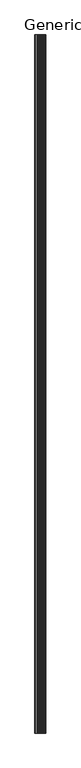
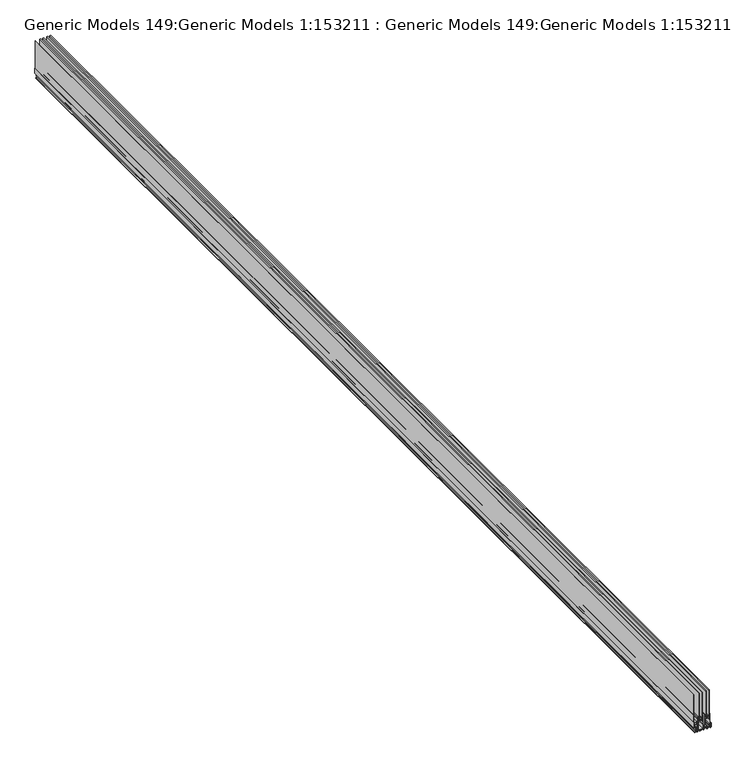
"""IFC4 building model written with IfcOpenShell, lengths in millimetres: proxy geometry, Generic Models 149:Generic Models 1:153211 : Generic Models 149:Generic Models 1:153211."""

from ifc_helpers import new_model, si_unit, frame, origin, place, context, project, spatial, polyline, outline, extrude, source, transform, mapped, element, save


def generic_models_149_generic_models_1_153211_generic_models_8e53df71(model_context):
    return source(origin(), model_context, "Body", "SweptSolid", [
        extrude(outline(polyline([(-6626.7463019, -5303.1974793), (-6626.7463019, 2583.5025207), (-6612.4164704, 2583.5025207), (-6612.4164704, -5303.1974793), (-6626.7463019, -5303.1974793)])), frame((0.0, 0.0, 55.1497405), z_axis=(0.0, 0.0, 1.0), x_axis=(1.0, 0.0, 0.0)), (0.0, 0.0, 1.0), 7.9798298),
        extrude(outline(polyline([(-6611.6227204, -5303.1974793), (-6611.6227204, 2583.5025207), (-6606.8813862, 2583.5025207), (-6606.8813862, -5303.1974793), (-6611.6227204, -5303.1974793)])), frame((0.0, 0.0, 54.3559905), z_axis=(0.0, 0.0, 1.0), x_axis=(1.0, 0.0, 0.0)), (0.0, 0.0, 1.0), 191.9290887),
        extrude(outline(polyline([(-6632.2813862, -5303.1974793), (-6632.2813862, 2583.5025207), (-6627.5400519, 2583.5025207), (-6627.5400519, -5303.1974793), (-6632.2813862, -5303.1974793)])), frame((0.0, 0.0, 54.3559905), z_axis=(0.0, 0.0, 1.0), x_axis=(1.0, 0.0, 0.0)), (0.0, 0.0, 1.0), 191.9290887),
        extrude(outline(polyline([(-6578.4016395, -5303.1974793), (-6578.4016395, 2583.5025207), (-6564.071808, 2583.5025207), (-6564.071808, -5303.1974793), (-6578.4016395, -5303.1974793)])), frame((0.0, 0.0, 55.1497405), z_axis=(0.0, 0.0, 1.0), x_axis=(1.0, 0.0, 0.0)), (0.0, 0.0, 1.0), 7.9798298),
        extrude(outline(polyline([(-15.24, -6644.7273792), (-15.24, -6643.4573766), (37.5919931, -6643.4573766), (37.5919931, -6646.5053852), (43.7726598, -6646.5053852), (43.7726598, -6664.8674677), (246.2850793, -6664.8674677), (246.2850793, -6665.6612177), (43.7726598, -6665.6612177), (43.7726598, -6667.2487177), (7.4338791, -6667.2487177), (4.8675216, -6657.1733817), (-15.2400103, -6657.1733817), (-15.2400103, -6655.9033792), (-2.2860103, -6655.9033792), (-2.2860103, -6644.7273792), (-15.24, -6644.7273792)]), holes=[polyline([(28.2786614, -6654.9720561), (26.5853256, -6654.9720561), (26.5853256, -6644.8120561), (-1.0160111, -6644.8120561), (-1.0160111, -6655.9033905), (5.8846955, -6655.9033905), (8.3602567, -6665.8940484), (12.1073187, -6665.8940484), (12.1073187, -6663.5233922), (13.3773204, -6663.5233922), (13.3773204, -6665.8940622), (36.3219905, -6665.8940622), (36.3219905, -6658.6973955), (42.5026598, -6658.6973955), (42.5026598, -6647.7753766), (36.3219931, -6647.7753766), (36.3219931, -6644.7273955), (28.2786614, -6644.7273955), (28.2786614, -6654.9720561)])]), frame((0.0, -5303.1974793, 0.0), z_axis=(0.0, 1.0, 0.0), x_axis=(0.0, 0.0, 1.0)), (0.0, 0.0, 1.0), 7886.7),
        extrude(outline(polyline([(-6563.278058, -5303.1974793), (-6563.278058, 2583.5025207), (-6558.5367238, 2583.5025207), (-6558.5367238, -5303.1974793), (-6563.278058, -5303.1974793)])), frame((0.0, 0.0, 54.3559905), z_axis=(0.0, 0.0, 1.0), x_axis=(1.0, 0.0, 0.0)), (0.0, 0.0, 1.0), 191.9290887),
        extrude(outline(polyline([(-6583.9367238, -5303.1974793), (-6583.9367238, 2583.5025207), (-6579.1953895, 2583.5025207), (-6579.1953895, -5303.1974793), (-6583.9367238, -5303.1974793)])), frame((0.0, 0.0, 54.3559905), z_axis=(0.0, 0.0, 1.0), x_axis=(1.0, 0.0, 0.0)), (0.0, 0.0, 1.0), 191.9290887),
        extrude(outline(polyline([(0.0, -6550.5780441), (-8.6360103, -6550.5780441), (-8.6360103, -6548.8000502), (-15.3674764, -6548.8000502), (-16.8486778, -6565.6487169), (-20.3200111, -6565.6487169), (-20.3200111, -6564.6327246), (-23.6220034, -6564.6327246), (-23.6220034, -6567.342058), (-22.6906701, -6568.1887246), (-22.0663514, -6569.1788543), (-21.6787466, -6570.1699246), (-21.5376159, -6571.1605246), (-21.6527194, -6572.1492432), (-22.0338174, -6573.1346691), (-22.6906701, -6574.1153913), (-23.6220034, -6575.0467246), (-23.6220034, -6577.7560502), (-20.320013, -6577.7560502), (-20.320013, -6576.7400502), (-17.8646796, -6576.7400502), (-17.8646796, -6580.1267169), (-20.320013, -6580.1267169), (-20.320013, -6602.1400502), (-22.860013, -6602.1400502), (-22.860013, -6605.0187169), (-20.4046796, -6605.0187169), (-20.4046796, -6634.1440502), (-22.860013, -6634.1440502), (-22.860013, -6637.0227169), (-20.4046796, -6637.0227169), (-20.4046796, -6639.4780502), (-27.7706796, -6639.4780502), (-27.7706796, -6649.2147169), (-23.7913463, -6649.2147169), (-23.7913463, -6651.1620502), (-27.7706796, -6651.1620502), (-27.7706796, -6660.6447169), (-31.750013, -6660.6447169), (-31.750013, -6654.2947169), (-30.1413463, -6654.2947169), (-30.1413463, -6641.5100502), (-31.750013, -6641.5100502), (-31.750013, -6637.0227169), (-25.2306796, -6637.0227169), (-25.2306796, -6633.2973835), (-22.860013, -6631.6810199), (-22.860013, -6624.1533905), (-31.7500155, -6624.1533905), (-31.7500155, -6621.6980571), (-29.8026822, -6621.6980571), (-28.0246822, -6620.6820571), (-27.4320198, -6621.2747195), (-26.3664552, -6621.6128724), (-25.1616557, -6621.5016454), (-24.4138082, -6620.853893), (-24.1056981, -6619.9009438), (-24.2201111, -6618.8741262), (-24.7398327, -6618.0047688), (-25.6476485, -6617.5242), (-26.4599658, -6617.5340508), (-27.4320181, -6617.8880511), (-28.0246847, -6618.4807177), (-30.1413514, -6617.2953844), (-29.3793514, -6616.2793844), (-28.528177, -6615.6312532), (-27.6236156, -6615.205372), (-26.6816597, -6614.9998594), (-25.718302, -6615.0128338), (-24.749535, -6615.2424137), (-23.7913514, -6615.6867177), (-22.8600181, -6616.4487177), (-22.8600181, -6607.4740511), (-25.2306847, -6605.7916425), (-25.2306847, -6598.9227177), (-31.7500181, -6598.9227177), (-31.7500181, -6596.5520511), (-23.6220181, -6596.5520511), (-23.6220181, -6580.1267177), (-25.9926847, -6578.4443091), (-25.9926847, -6575.8087177), (-31.7500181, -6575.8087177), (-31.7500181, -6573.4380511), (-30.0566847, -6573.4380511), (-28.0246847, -6572.2527177), (-27.4320181, -6572.9300588), (-26.4101923, -6573.2529926), (-25.2207414, -6573.1319292), (-24.4457934, -6572.4847749), (-24.0882255, -6571.5370539), (-24.1509152, -6570.5142905), (-24.6367399, -6569.6420089), (-25.5485767, -6569.1457332), (-26.3945623, -6569.135145), (-27.4320181, -6569.4587255), (-28.0246847, -6570.1360588), (-30.1413514, -6568.8660588), (-29.3793514, -6567.9347255), (-28.3633514, -6567.1727255), (-27.2626847, -6566.7493922), (-25.9926847, -6566.5800588), (-25.9926847, -6562.2620502), (-18.913985, -6562.2620502), (-17.8105346, -6548.8000441), (-26.924, -6548.8000441), (-26.924, -6551.1707108), (-29.3793333, -6551.1707108), (-29.3793333, -6552.7793775), (-31.75, -6552.7793775), (-31.75, -6548.8000441), (-29.3793333, -6548.8000441), (-29.3793333, -6546.3447108), (0.0, -6546.3447108), (0.0, -6550.5780441)])), frame((0.0, -5303.1974793, 0.0), z_axis=(0.0, 1.0, 0.0), x_axis=(0.0, 0.0, 1.0)), (0.0, 0.0, 1.0), 7886.7),
        extrude(outline(polyline([(-13.8853402, -6587.2387142), (-11.5146736, -6585.0373809), (-11.5146736, -6581.1427117), (-4.5720042, -6581.1427117), (-4.5720042, -6586.0533905), (32.3426624, -6586.0533905), (32.3426624, -6582.8360571), (33.9513291, -6582.8360571), (33.9513291, -6586.0533792), (48.8526537, -6586.0533792), (49.6993204, -6585.8840458), (50.545987, -6585.3760458), (51.053987, -6584.5293792), (51.2233204, -6583.6827125), (51.2233204, -6577.3327125), (51.0539905, -6576.5707125), (49.7937115, -6575.3596656), (48.8208346, -6575.2246403), (47.8761103, -6575.6274864), (47.0746572, -6576.5707125), (46.9053239, -6577.3327125), (46.9053239, -6579.9573792), (45.0426572, -6579.9573792), (45.0426572, -6573.5227125), (47.1593239, -6572.3373792), (47.6673239, -6572.9300571), (48.9341881, -6573.370951), (49.7440381, -6573.2555999), (50.445459, -6572.8014428), (50.9693239, -6571.9987238), (51.1386572, -6571.2367238), (50.969335, -6570.4747255), (50.1126338, -6569.4019675), (49.3483574, -6569.1184329), (48.5102155, -6569.1688264), (47.667335, -6569.5433922), (47.159335, -6570.1360588), (45.0426684, -6568.9507091), (45.0426684, -6562.5160425), (46.905335, -6562.5160425), (46.905335, -6565.1407091), (47.0746537, -6565.9027134), (48.3377549, -6567.1150146), (49.3109454, -6567.2487856), (50.254729, -6566.8443135), (51.053987, -6565.9027134), (51.2233308, -6565.1407134), (51.2233308, -6558.7907238), (51.0539975, -6557.8593905), (50.5459975, -6557.0973905), (49.6993308, -6556.5893905), (48.8526641, -6556.4200571), (33.9513308, -6556.4200571), (33.9513308, -6559.6373905), (32.3426641, -6559.6373905), (32.3426641, -6556.4200571), (-4.5720034, -6556.4200571), (-4.5720034, -6561.3307228), (-10.1600034, -6561.3307228), (-10.1600034, -6554.0493878), (75.0146624, -6554.0493878), (75.0146624, -6556.4200467), (55.964665, -6556.4200467), (55.0333316, -6556.58938), (54.2713316, -6557.09738), (53.7633316, -6557.85938), (53.593988, -6558.7907134), (53.593988, -6583.6827238), (53.7633213, -6584.5293905), (54.2713213, -6585.3760571), (55.0333213, -6585.8840571), (55.9646547, -6586.0533905), (75.0146547, -6586.0533905), (75.0146547, -6588.4240571), (-12.7483988, -6588.4240571), (-15.7480069, -6591.0487142), (-17.6953402, -6593.0807142), (-19.3040069, -6595.2820475), (-17.8646736, -6592.3187142), (-16.0020069, -6589.6940475), (-13.8853402, -6587.2387142)])), frame((0.0, -5303.1974793, 0.0), z_axis=(0.0, 1.0, 0.0), x_axis=(0.0, 0.0, 1.0)), (0.0, 0.0, 1.0), 7886.7),
        extrude(outline(polyline([(32.3426641, -6604.764716), (-22.0133376, -6604.764716), (-22.0133376, -6602.3940502), (75.0146624, -6602.3940502), (75.0146624, -6604.7647091), (55.964665, -6604.7647091), (55.0333316, -6604.9340425), (54.2713316, -6605.4420425), (53.7633316, -6606.2040425), (53.593988, -6607.1353758), (53.593988, -6632.0273862), (53.7633213, -6632.8740529), (54.2713213, -6633.7207196), (55.0333213, -6634.2287196), (55.9646547, -6634.3980529), (75.0146624, -6634.3980529), (75.0146624, -6636.768715), (-22.0133376, -6636.768715), (-22.0133376, -6634.3980614), (32.3426624, -6634.3980614), (32.3426624, -6631.1807196), (33.9513291, -6631.1807196), (33.9513291, -6634.3980416), (48.8526537, -6634.3980416), (49.6993204, -6634.2287083), (50.545987, -6633.7207083), (51.053987, -6632.8740416), (51.2233204, -6632.0273749), (51.2233204, -6625.6773749), (51.0539905, -6624.9153749), (49.7937115, -6623.704328), (48.8208346, -6623.5693027), (47.8761103, -6623.9721488), (47.0746572, -6624.9153749), (46.9053239, -6625.6773749), (46.9053239, -6628.3020416), (45.0426572, -6628.3020416), (45.0426572, -6621.8673749), (47.1593239, -6620.6820416), (47.6673239, -6621.2747196), (48.9341881, -6621.7156134), (49.7440381, -6621.6002623), (50.445459, -6621.1461052), (50.9693239, -6620.3433862), (51.1386572, -6619.5813862), (50.969335, -6618.8193879), (50.1126338, -6617.7466299), (49.3483574, -6617.4630953), (48.5102155, -6617.5134888), (47.667335, -6617.8880546), (47.159335, -6618.4807213), (45.0426684, -6617.2953716), (45.0426684, -6610.8607049), (46.905335, -6610.8607049), (46.905335, -6613.4853716), (47.0746537, -6614.2473758), (48.3377549, -6615.459677), (49.3109454, -6615.593448), (50.254729, -6615.188976), (51.053987, -6614.2473758), (51.2233308, -6613.4853758), (51.2233308, -6607.1353862), (51.0539975, -6606.2040529), (50.5459975, -6605.4420529), (49.6993308, -6604.9340529), (48.8526641, -6604.7647196), (33.9513308, -6604.7647196), (33.9513308, -6607.9820529), (32.3426641, -6607.9820529), (32.3426641, -6604.764716)])), frame((0.0, -5303.1974793, 0.0), z_axis=(0.0, 1.0, 0.0), x_axis=(0.0, 0.0, 1.0)), (0.0, 0.0, 1.0), 7886.7),
    ])


if __name__ == "__main__":
    model = new_model("IFC4")
    model_context = context("Model", 3, world=origin())
    ifc_project = project(units=[si_unit("LENGTHUNIT", "METRE", prefix="MILLI")], contexts=[model_context])
    site = spatial("IfcSite", under=ifc_project)
    building = spatial("IfcBuilding", under=site)
    placement = place(None, origin())
    generic_models_149_generic_models_1_153211_generic_models_shape = generic_models_149_generic_models_1_153211_generic_models_8e53df71(model_context)
    element("IfcBuildingElementProxy", 1, Name="Generic Models 149:Generic Models 1:153211 : Generic Models 149:Generic Models 1:153211", ObjectType="Generic Models 149:Generic Models 1:153211 : Generic Models 149:Generic Models 1:153211", at=placement, inside=building, context=model_context, shape_type="MappedRepresentation", body=[
        mapped(generic_models_149_generic_models_1_153211_generic_models_shape, transform((0.0, 0.0, 0.0), x_axis=(1.0, 0.0, 0.0), y_axis=(0.0, 1.0, 0.0), z_axis=(0.0, 0.0, 1.0))),
    ])
    save(model, "model.ifc")

# Revit data of these elements
# Type "Generic Models 149:Generic Models 1:153211 : Generic Models 149:Generic Models 1:153211"
#   NameOverride = "Generic Models 149:Generic Models 1:153211"
#   ObjectTypeOverride = "Generic Models 149:Generic Models 1"
#   Reference = "Generic Models 1"
#   Category = "Generic Models"
#   Tag = "153211"
# Element 1 (IfcBuildingElementProxy, "Generic Models 149:Generic Models 1:153211 : Generic Models 149:Generic Models 1:153211")
#   Materials on its faces: "_SIDING DOOR PER SCHEDULE 11160"
# Materials
#   "_SIDING DOOR PER SCHEDULE 11160": class "Unassigned", colour RGB 255 255 255, transparency 0
